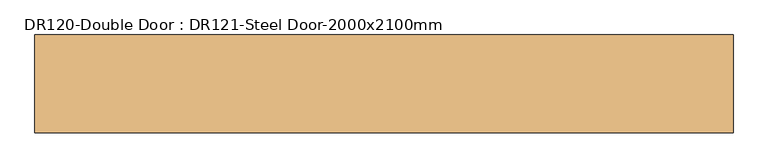
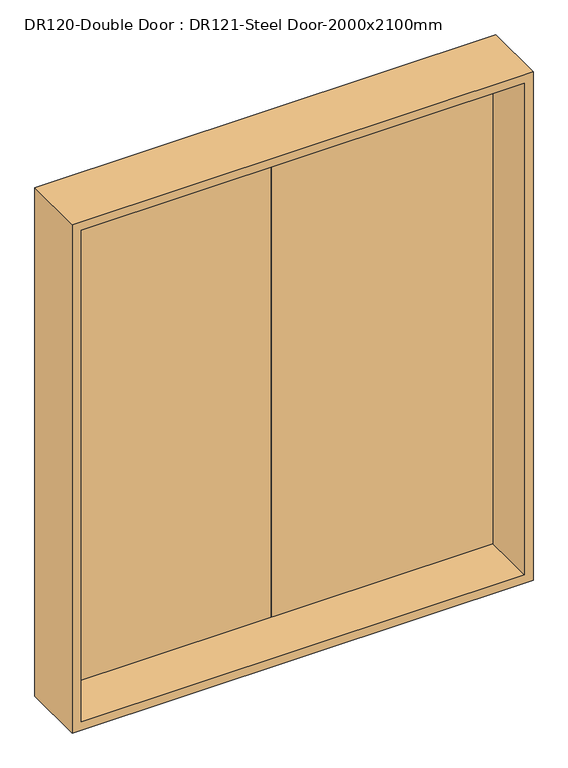
"""IFC4 building model written with IfcOpenShell, lengths in millimetres: door geometry, DR120-Double Door : DR121-Steel Door-2000x2100mm."""

import ifcopenshell
import ifcopenshell.guid

model = None  # the IFC model being written
_history = None  # IfcOwnerHistory: only IFC2X3 demands one
_inside = {}  # id of a spatial element -> (the spatial element, [elements in it])
_under = {}  # id of a project, library or spatial element -> (it, [spatial elements below it])
_declared = {}  # id of a project -> (the project, [libraries it declares])
_typed = {}  # id of a type object -> (the type object, [elements of that type])
_made_of = {}  # id of a material, layer set ... -> (it, [elements and type objects made of it])


def new_model(schema):
    """Start an empty IFC model of exactly this schema.

    Asked for "IFC4X3", IfcOpenShell would pick the latest addendum, in which some entities
    have other attributes; the version numbers below select the first issue.
    IFC2X3 requires an IfcOwnerHistory on every rooted entity: one is made here for all.
    """
    global model, _history
    if schema == "IFC4X3":
        model = ifcopenshell.file(schema_version=(4, 3, 0, 0))
    else:
        model = ifcopenshell.file(schema=schema)
    _inside.clear()
    _under.clear()
    _declared.clear()
    _typed.clear()
    _made_of.clear()
    _history = None
    if model.schema == "IFC2X3":
        org = make("IfcOrganization", Name="unknown")
        user = make(
            "IfcPersonAndOrganization",
            ThePerson=make("IfcPerson", FamilyName="unknown"),
            TheOrganization=org,
        )
        app = make(
            "IfcApplication",
            ApplicationDeveloper=org,
            Version="unknown",
            ApplicationFullName="unknown",
            ApplicationIdentifier="unknown",
        )
        _history = make(
            "IfcOwnerHistory",
            OwningUser=user,
            OwningApplication=app,
            ChangeAction="ADDED",
            CreationDate=0,
        )
    return model


def make(cls, **values):
    """One entity of the class cls with the attributes given. An attribute that is None is left unset."""
    return model.create_entity(
        cls, **{name: value for name, value in values.items() if value is not None}
    )


def rooted(cls, **values):
    """An entity with a GlobalId (a new one), such as an element, a storey or a relation."""
    return make(cls, GlobalId=ifcopenshell.guid.new(), OwnerHistory=_history, **values)


def si_unit(unit_type, name, prefix=None):
    """IfcSIUnit, for example si_unit("LENGTHUNIT", "METRE", prefix="MILLI")."""
    return make("IfcSIUnit", UnitType=unit_type, Prefix=prefix, Name=name)


def assignment(units):
    """IfcUnitAssignment: the units of a project."""
    return None if units is None else make("IfcUnitAssignment", Units=units)


def point(xyz):
    """IfcCartesianPoint."""
    return None if xyz is None else make("IfcCartesianPoint", Coordinates=xyz)


def direction(xyz):
    """IfcDirection."""
    return None if xyz is None else make("IfcDirection", DirectionRatios=xyz)


def frame(location, z_axis=None, x_axis=None):
    """IfcAxis2Placement3D, a coordinate frame: its origin and axes. An axis left out is left unset."""
    return make(
        "IfcAxis2Placement3D",
        Location=point(location),
        Axis=direction(z_axis),
        RefDirection=direction(x_axis),
    )


def origin():
    """The frame at (0, 0, 0) with its axes left unset."""
    return frame((0.0, 0.0, 0.0))


def place(relative_to, where):
    """IfcLocalPlacement: puts the frame where relative to a parent placement (None: the world)."""
    return make(
        "IfcLocalPlacement", PlacementRelTo=relative_to, RelativePlacement=where
    )


def context(
    kind, dimensions, precision=None, world=None, true_north=None, identifier=None
):
    """IfcGeometricRepresentationContext, for example the 3D "Model" context."""
    return make(
        "IfcGeometricRepresentationContext",
        ContextIdentifier=identifier,
        ContextType=kind,
        CoordinateSpaceDimension=dimensions,
        Precision=precision,
        WorldCoordinateSystem=world,
        TrueNorth=true_north,
    )


def project(units=None, contexts=None):
    """IfcProject with its units and contexts."""
    return rooted(
        "IfcProject",
        Name="project",
        RepresentationContexts=contexts,
        UnitsInContext=assignment(units),
    )


def spatial(cls, under=None, at=None, **own):
    """A site, building, storey or space (cls), placed at a placement, below another one or the project."""
    s = rooted(cls, ObjectPlacement=at, **own)
    if under is not None:
        _under.setdefault(under.id(), (under, []))[1].append(s)
    return s


def polyline(points):
    """IfcPolyline through the points."""
    return make("IfcPolyline", Points=[point(p) for p in points])


def outline(outer, holes=None, kind="AREA"):
    """IfcArbitraryClosedProfileDef: a profile drawn as a closed curve; with holes, ...WithVoids."""
    if holes is None:
        return make("IfcArbitraryClosedProfileDef", ProfileType=kind, OuterCurve=outer)
    return make(
        "IfcArbitraryProfileDefWithVoids",
        ProfileType=kind,
        OuterCurve=outer,
        InnerCurves=holes,
    )


def extrude(swept, where, along, depth):
    """IfcExtrudedAreaSolid: the profile swept, set in the frame where, extruded along a direction by depth."""
    return make(
        "IfcExtrudedAreaSolid",
        SweptArea=swept,
        Position=where,
        ExtrudedDirection=direction(along),
        Depth=depth,
    )


def faces_of(points, faces, orient=None, outer=None):
    """IfcFace entities. A face is a list of loops; a loop is a list of indices into points, from 0.

    orient and outer hold one flag for each loop. By default every Orientation is true, the
    first loop of a face is its IfcFaceOuterBound and the others are IfcFaceBound.
    """
    made = []
    for i, loops in enumerate(faces):
        bounds = []
        for j, loop in enumerate(loops):
            is_outer = j == 0 if outer is None else outer[i][j]
            bounds.append(
                make(
                    "IfcFaceOuterBound" if is_outer else "IfcFaceBound",
                    Bound=make("IfcPolyLoop", Polygon=[points[k] for k in loop]),
                    Orientation=True if orient is None else orient[i][j],
                )
            )
        made.append(make("IfcFace", Bounds=bounds))
    return made


def faceted_brep(points, faces, orient=None, outer=None, voids=None):
    """IfcFacetedBrep: a solid bounded by flat faces; with voids (closed shells), ...WithVoids."""
    shared = [point(p) for p in points]
    hull = make("IfcClosedShell", CfsFaces=faces_of(shared, faces, orient, outer))
    if voids is None:
        return make("IfcFacetedBrep", Outer=hull)
    return make(
        "IfcFacetedBrepWithVoids",
        Outer=hull,
        Voids=[
            make(cls, CfsFaces=faces_of(shared, fs, o, b)) for cls, fs, o, b in voids
        ],
    )


def shape(context_of_items, identifier, shape_type, items):
    """IfcShapeRepresentation: the items that make up one representation, for example the "Body"."""
    return make(
        "IfcShapeRepresentation",
        ContextOfItems=context_of_items,
        RepresentationIdentifier=identifier,
        RepresentationType=shape_type,
        Items=items,
    )


def source(mapping_origin, context_of_items, identifier, shape_type, items):
    """IfcRepresentationMap: a shape defined once, which mapped items show again and again."""
    return make(
        "IfcRepresentationMap",
        MappingOrigin=mapping_origin,
        MappedRepresentation=shape(context_of_items, identifier, shape_type, items),
    )


def transform(
    local_origin,
    x_axis=None,
    y_axis=None,
    z_axis=None,
    scale=None,
    scale2=None,
    scale3=None,
    uniform=True,
):
    """IfcCartesianTransformationOperator3D, or its non-uniform kind. x_axis, y_axis, z_axis: its Axis1, 2, 3."""
    if uniform:
        return make(
            "IfcCartesianTransformationOperator3D",
            Axis1=direction(x_axis),
            Axis2=direction(y_axis),
            LocalOrigin=point(local_origin),
            Scale=scale,
            Axis3=direction(z_axis),
        )
    return make(
        "IfcCartesianTransformationOperator3DnonUniform",
        Axis1=direction(x_axis),
        Axis2=direction(y_axis),
        LocalOrigin=point(local_origin),
        Scale=scale,
        Axis3=direction(z_axis),
        Scale2=scale2,
        Scale3=scale3,
    )


def mapped(mapping_source, mapping_target):
    """IfcMappedItem: shows the shape of a source again, moved by a transform."""
    return make(
        "IfcMappedItem", MappingSource=mapping_source, MappingTarget=mapping_target
    )


def made_of(thing, what):
    """Note that an element or type object is made of a material, layer set ...; save() writes the relation."""
    if what is not None:
        _made_of.setdefault(what.id(), (what, []))[1].append(thing)
    return thing


def element(
    cls,
    number,
    at=None,
    inside=None,
    cuts=None,
    type_object=None,
    material=None,
    context=None,
    identifier="Body",
    shape_type=None,
    held_by="IfcProductDefinitionShape",
    body=None,
    shapes=None,
    **own,
):
    """One element of the class cls, such as IfcWall. Its Tag is "e" and its number.

    at: its placement. inside: the storey or other place that contains it. cuts: it is an
    opening in that element (IfcRelVoidsElement). A single representation is given by context,
    identifier, shape_type and body (its items); several are given by shapes. held_by: the class
    of the entity that holds the representations. save() writes the other relations.
    """
    e = rooted(cls, Tag="e%d" % number, ObjectPlacement=at, **own)
    if body is not None:
        shapes = [shape(context, identifier, shape_type, body)]
    if shapes is not None:
        e.Representation = make(held_by, Representations=shapes)
    if inside is not None:
        _inside.setdefault(inside.id(), (inside, []))[1].append(e)
    if cuts is not None:
        rooted(
            "IfcRelVoidsElement", RelatingBuildingElement=cuts, RelatedOpeningElement=e
        )
    if type_object is not None:
        _typed.setdefault(type_object.id(), (type_object, []))[1].append(e)
    return made_of(e, material)


def aggregate(whole, parts):
    """IfcRelAggregates: a whole, such as a stair, and the parts it consists of."""
    return rooted("IfcRelAggregates", RelatingObject=whole, RelatedObjects=parts)


def save(model, path):
    """Write the relations noted so far, then the file.

    IfcRelAggregates (storeys below a building ...), IfcRelContainedInSpatialStructure (elements
    in a storey), IfcRelDefinesByType, IfcRelAssociatesMaterial and IfcRelDeclares: one each for
    every whole, place, type object, material and project.
    """
    for whole, parts in _under.values():
        aggregate(whole, parts)
    for where, things in _inside.values():
        rooted(
            "IfcRelContainedInSpatialStructure",
            RelatedElements=things,
            RelatingStructure=where,
        )
    for kind, things in _typed.values():
        rooted("IfcRelDefinesByType", RelatedObjects=things, RelatingType=kind)
    for what, things in _made_of.values():
        rooted("IfcRelAssociatesMaterial", RelatedObjects=things, RelatingMaterial=what)
    for by, libraries in _declared.values():
        rooted("IfcRelDeclares", RelatingContext=by, RelatedDefinitions=libraries)
    model.write(path)


def dr120_double_door_dr121_steel_door_2000x2100mm_b0f5a95a(model_context):
    return source(origin(), model_context, "Body", "SolidModel", [
        extrude(outline(polyline([(880.0, 86.0), (0.0, 86.0), (0.0, 126.0), (880.0, 126.0), (880.0, 86.0)])), frame((0.0, 0.0, 20.0), z_axis=(0.0, 0.0, 1.0), x_axis=(1.0, 0.0, 0.0)), (0.0, 0.0, 1.0), 2060.0),
        extrude(outline(polyline([(0.0, 86.0), (-880.0, 86.0), (-880.0, 126.0), (0.0, 126.0), (0.0, 86.0)])), frame((0.0, 0.0, 20.0), z_axis=(0.0, 0.0, 1.0), x_axis=(1.0, 0.0, 0.0)), (0.0, 0.0, 1.0), 2060.0),
        faceted_brep([(900.0, -126.0, 2100.0), (900.0, 126.0, 2100.0), (-900.0, 126.0, 2100.0), (-900.0, -126.0, 2100.0), (865.0, 86.0, 2065.0), (865.0, -126.0, 2065.0), (-865.0, -126.0, 2065.0), (-865.0, 86.0, 2065.0), (880.0, 126.0, 2080.0), (880.0, 86.0, 2080.0), (-880.0, 86.0, 2080.0), (-880.0, 126.0, 2080.0), (-900.0, 126.0, 0.0), (-900.0, -126.0, 0.0), (-865.0, -126.0, 35.0), (-865.0, 86.0, 35.0), (-880.0, 86.0, 20.0), (-880.0, 126.0, 20.0), (900.0, 126.0, 0.0), (880.0, 126.0, 20.0), (900.0, -126.0, 0.0), (865.0, -126.0, 35.0), (865.0, 86.0, 35.0), (880.0, 86.0, 20.0)], [[[0, 1, 2, 3]], [[4, 5, 6, 7]], [[8, 9, 10, 11]], [[3, 2, 12, 13]], [[7, 6, 14, 15]], [[11, 10, 16, 17]], [[18, 12, 2, 1], [8, 11, 17, 19]], [[13, 12, 18, 20]], [[0, 3, 13, 20], [21, 14, 6, 5]], [[15, 14, 21, 22]], [[23, 16, 10, 9], [4, 7, 15, 22]], [[17, 16, 23, 19]], [[20, 18, 1, 0]], [[22, 21, 5, 4]], [[19, 23, 9, 8]]]),
    ])


if __name__ == "__main__":
    model = new_model("IFC4")
    model_context = context("Model", 3, world=origin())
    ifc_project = project(units=[si_unit("LENGTHUNIT", "METRE", prefix="MILLI")], contexts=[model_context])
    site = spatial("IfcSite", under=ifc_project)
    building = spatial("IfcBuilding", under=site)
    placement = place(None, origin())
    dr120_double_door_dr121_steel_door_2000x2100mm_shape = dr120_double_door_dr121_steel_door_2000x2100mm_b0f5a95a(model_context)
    element("IfcDoor", 1, ObjectType="DR120-Double Door : DR121-Steel Door-2000x2100mm", at=placement, inside=building, context=model_context, shape_type="MappedRepresentation", body=[
        mapped(dr120_double_door_dr121_steel_door_2000x2100mm_shape, transform((0.0, 0.0, 0.0), x_axis=(1.0, 0.0, 0.0), y_axis=(0.0, 1.0, 0.0), z_axis=(0.0, 0.0, 1.0))),
    ])
    save(model, "model.ifc")

# Revit data of these elements
# Type "DR120-Double Door : DR121-Steel Door-2000x2100mm"
#   Type Mark = "SD"
#   프레임 = ""
#   철물 = ""
#   유리/마감 = ""
#   위치/개소 = ""
#   부호 = "1/SD"
#   문번호 = ""
#   문기호 = "SD"
#   Analytic Construction = "<None>"
#   Height = 2100 mm
#   Width = 1800 mm
#   Define Thermal Properties by = 1
#   문 틀 = A04AQ098-00003_Steel Door_non FP_double
#   문 = 문
#   Function = (empty or 0)
#   Assembly Code = ""
#   Wall Closure = (empty or 0)
# Element 1 (IfcDoor, "DR120-Double Door : DR121-Steel Door-2000x2100mm")
#   Materials on its faces: "A04AQ098-00003_Steel Door_non FP_double", "문"
# Materials
#   "A04AQ098-00003_Steel Door_non FP_double": class "금속", colour RGB 247 247 247, transparency 0, Description = "Steel Door", W00) Work Master Code = "A04AQ098-00003", W01) Work Master_Lv1 = "Finishing Work", W02) Work Master_Lv2 = "Door & Window Work", W03) Work Master_Spec.1 = "Steel Door w/ Steel Frame", W04) Work Master_Spec.2 = "Fire Protective Rating: N/A, Double Door", W05) Work Master_Spec.3 = "w/ Hardware & Accessories", Cost = 0
#   "문": class "다양한", colour RGB 247 247 247, transparency 0
